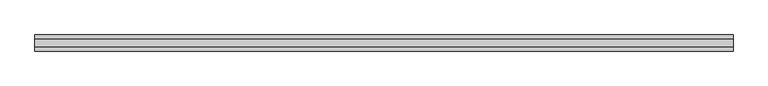
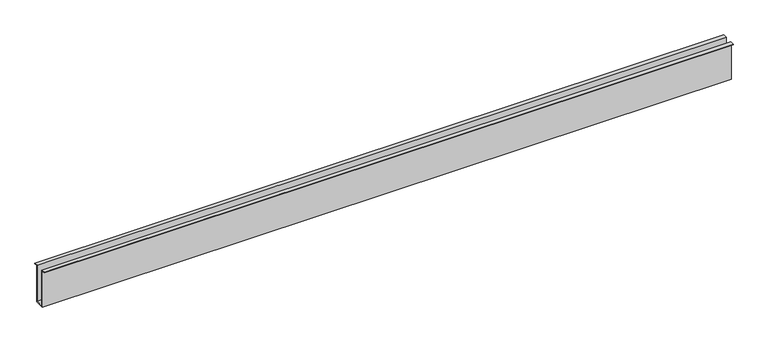
"""IFC4 building model written with IfcOpenShell, lengths in millimetres: railing geometry, ML_Perfil U de embutir1 : ML_Perfil U de embutir."""

import ifcopenshell
import ifcopenshell.guid

model = None  # the IFC model being written
_history = None  # IfcOwnerHistory: only IFC2X3 demands one
_inside = {}  # id of a spatial element -> (the spatial element, [elements in it])
_under = {}  # id of a project, library or spatial element -> (it, [spatial elements below it])
_declared = {}  # id of a project -> (the project, [libraries it declares])
_typed = {}  # id of a type object -> (the type object, [elements of that type])
_made_of = {}  # id of a material, layer set ... -> (it, [elements and type objects made of it])


def new_model(schema):
    """Start an empty IFC model of exactly this schema.

    Asked for "IFC4X3", IfcOpenShell would pick the latest addendum, in which some entities
    have other attributes; the version numbers below select the first issue.
    IFC2X3 requires an IfcOwnerHistory on every rooted entity: one is made here for all.
    """
    global model, _history
    if schema == "IFC4X3":
        model = ifcopenshell.file(schema_version=(4, 3, 0, 0))
    else:
        model = ifcopenshell.file(schema=schema)
    _inside.clear()
    _under.clear()
    _declared.clear()
    _typed.clear()
    _made_of.clear()
    _history = None
    if model.schema == "IFC2X3":
        org = make("IfcOrganization", Name="unknown")
        user = make(
            "IfcPersonAndOrganization",
            ThePerson=make("IfcPerson", FamilyName="unknown"),
            TheOrganization=org,
        )
        app = make(
            "IfcApplication",
            ApplicationDeveloper=org,
            Version="unknown",
            ApplicationFullName="unknown",
            ApplicationIdentifier="unknown",
        )
        _history = make(
            "IfcOwnerHistory",
            OwningUser=user,
            OwningApplication=app,
            ChangeAction="ADDED",
            CreationDate=0,
        )
    return model


def make(cls, **values):
    """One entity of the class cls with the attributes given. An attribute that is None is left unset."""
    return model.create_entity(
        cls, **{name: value for name, value in values.items() if value is not None}
    )


def rooted(cls, **values):
    """An entity with a GlobalId (a new one), such as an element, a storey or a relation."""
    return make(cls, GlobalId=ifcopenshell.guid.new(), OwnerHistory=_history, **values)


def si_unit(unit_type, name, prefix=None):
    """IfcSIUnit, for example si_unit("LENGTHUNIT", "METRE", prefix="MILLI")."""
    return make("IfcSIUnit", UnitType=unit_type, Prefix=prefix, Name=name)


def assignment(units):
    """IfcUnitAssignment: the units of a project."""
    return None if units is None else make("IfcUnitAssignment", Units=units)


def point(xyz):
    """IfcCartesianPoint."""
    return None if xyz is None else make("IfcCartesianPoint", Coordinates=xyz)


def direction(xyz):
    """IfcDirection."""
    return None if xyz is None else make("IfcDirection", DirectionRatios=xyz)


def frame(location, z_axis=None, x_axis=None):
    """IfcAxis2Placement3D, a coordinate frame: its origin and axes. An axis left out is left unset."""
    return make(
        "IfcAxis2Placement3D",
        Location=point(location),
        Axis=direction(z_axis),
        RefDirection=direction(x_axis),
    )


def origin():
    """The frame at (0, 0, 0) with its axes left unset."""
    return frame((0.0, 0.0, 0.0))


def place(relative_to, where):
    """IfcLocalPlacement: puts the frame where relative to a parent placement (None: the world)."""
    return make(
        "IfcLocalPlacement", PlacementRelTo=relative_to, RelativePlacement=where
    )


def context(
    kind, dimensions, precision=None, world=None, true_north=None, identifier=None
):
    """IfcGeometricRepresentationContext, for example the 3D "Model" context."""
    return make(
        "IfcGeometricRepresentationContext",
        ContextIdentifier=identifier,
        ContextType=kind,
        CoordinateSpaceDimension=dimensions,
        Precision=precision,
        WorldCoordinateSystem=world,
        TrueNorth=true_north,
    )


def project(units=None, contexts=None):
    """IfcProject with its units and contexts."""
    return rooted(
        "IfcProject",
        Name="project",
        RepresentationContexts=contexts,
        UnitsInContext=assignment(units),
    )


def spatial(cls, under=None, at=None, **own):
    """A site, building, storey or space (cls), placed at a placement, below another one or the project."""
    s = rooted(cls, ObjectPlacement=at, **own)
    if under is not None:
        _under.setdefault(under.id(), (under, []))[1].append(s)
    return s


def polyline(points):
    """IfcPolyline through the points."""
    return make("IfcPolyline", Points=[point(p) for p in points])


def outline(outer, holes=None, kind="AREA"):
    """IfcArbitraryClosedProfileDef: a profile drawn as a closed curve; with holes, ...WithVoids."""
    if holes is None:
        return make("IfcArbitraryClosedProfileDef", ProfileType=kind, OuterCurve=outer)
    return make(
        "IfcArbitraryProfileDefWithVoids",
        ProfileType=kind,
        OuterCurve=outer,
        InnerCurves=holes,
    )


def extrude(swept, where, along, depth):
    """IfcExtrudedAreaSolid: the profile swept, set in the frame where, extruded along a direction by depth."""
    return make(
        "IfcExtrudedAreaSolid",
        SweptArea=swept,
        Position=where,
        ExtrudedDirection=direction(along),
        Depth=depth,
    )


def shape(context_of_items, identifier, shape_type, items):
    """IfcShapeRepresentation: the items that make up one representation, for example the "Body"."""
    return make(
        "IfcShapeRepresentation",
        ContextOfItems=context_of_items,
        RepresentationIdentifier=identifier,
        RepresentationType=shape_type,
        Items=items,
    )


def source(mapping_origin, context_of_items, identifier, shape_type, items):
    """IfcRepresentationMap: a shape defined once, which mapped items show again and again."""
    return make(
        "IfcRepresentationMap",
        MappingOrigin=mapping_origin,
        MappedRepresentation=shape(context_of_items, identifier, shape_type, items),
    )


def transform(
    local_origin,
    x_axis=None,
    y_axis=None,
    z_axis=None,
    scale=None,
    scale2=None,
    scale3=None,
    uniform=True,
):
    """IfcCartesianTransformationOperator3D, or its non-uniform kind. x_axis, y_axis, z_axis: its Axis1, 2, 3."""
    if uniform:
        return make(
            "IfcCartesianTransformationOperator3D",
            Axis1=direction(x_axis),
            Axis2=direction(y_axis),
            LocalOrigin=point(local_origin),
            Scale=scale,
            Axis3=direction(z_axis),
        )
    return make(
        "IfcCartesianTransformationOperator3DnonUniform",
        Axis1=direction(x_axis),
        Axis2=direction(y_axis),
        LocalOrigin=point(local_origin),
        Scale=scale,
        Axis3=direction(z_axis),
        Scale2=scale2,
        Scale3=scale3,
    )


def mapped(mapping_source, mapping_target):
    """IfcMappedItem: shows the shape of a source again, moved by a transform."""
    return make(
        "IfcMappedItem", MappingSource=mapping_source, MappingTarget=mapping_target
    )


def made_of(thing, what):
    """Note that an element or type object is made of a material, layer set ...; save() writes the relation."""
    if what is not None:
        _made_of.setdefault(what.id(), (what, []))[1].append(thing)
    return thing


def element(
    cls,
    number,
    at=None,
    inside=None,
    cuts=None,
    type_object=None,
    material=None,
    context=None,
    identifier="Body",
    shape_type=None,
    held_by="IfcProductDefinitionShape",
    body=None,
    shapes=None,
    **own,
):
    """One element of the class cls, such as IfcWall. Its Tag is "e" and its number.

    at: its placement. inside: the storey or other place that contains it. cuts: it is an
    opening in that element (IfcRelVoidsElement). A single representation is given by context,
    identifier, shape_type and body (its items); several are given by shapes. held_by: the class
    of the entity that holds the representations. save() writes the other relations.
    """
    e = rooted(cls, Tag="e%d" % number, ObjectPlacement=at, **own)
    if body is not None:
        shapes = [shape(context, identifier, shape_type, body)]
    if shapes is not None:
        e.Representation = make(held_by, Representations=shapes)
    if inside is not None:
        _inside.setdefault(inside.id(), (inside, []))[1].append(e)
    if cuts is not None:
        rooted(
            "IfcRelVoidsElement", RelatingBuildingElement=cuts, RelatedOpeningElement=e
        )
    if type_object is not None:
        _typed.setdefault(type_object.id(), (type_object, []))[1].append(e)
    return made_of(e, material)


def aggregate(whole, parts):
    """IfcRelAggregates: a whole, such as a stair, and the parts it consists of."""
    return rooted("IfcRelAggregates", RelatingObject=whole, RelatedObjects=parts)


def save(model, path):
    """Write the relations noted so far, then the file.

    IfcRelAggregates (storeys below a building ...), IfcRelContainedInSpatialStructure (elements
    in a storey), IfcRelDefinesByType, IfcRelAssociatesMaterial and IfcRelDeclares: one each for
    every whole, place, type object, material and project.
    """
    for whole, parts in _under.values():
        aggregate(whole, parts)
    for where, things in _inside.values():
        rooted(
            "IfcRelContainedInSpatialStructure",
            RelatedElements=things,
            RelatingStructure=where,
        )
    for kind, things in _typed.values():
        rooted("IfcRelDefinesByType", RelatedObjects=things, RelatingType=kind)
    for what, things in _made_of.values():
        rooted("IfcRelAssociatesMaterial", RelatedObjects=things, RelatingMaterial=what)
    for by, libraries in _declared.values():
        rooted("IfcRelDeclares", RelatingContext=by, RelatedDefinitions=libraries)
    model.write(path)


def railing_4d275163(model_context):
    return source(origin(), model_context, "Body", "SweptSolid", [
        extrude(outline(polyline([(1832.4523952, 3702.0), (1832.4523952, 3594.0), (1856.4523952, 3594.0), (1856.4523952, 3702.0), (1866.9523952, 3702.0), (1866.9523952, 3700.0), (1858.4523952, 3700.0), (1858.4523952, 3592.0), (1830.4523952, 3592.0), (1830.4523952, 3700.0), (1821.9523952, 3700.0), (1821.9523952, 3702.0), (1832.4523952, 3702.0)])), frame((-12226.1487231, 0.0, 0.0), z_axis=(1.0, 0.0, 0.0), x_axis=(0.0, 1.0, 0.0)), (0.0, 0.0, 1.0), 1950.0),
    ])


if __name__ == "__main__":
    model = new_model("IFC4")
    model_context = context("Model", 3, world=origin())
    ifc_project = project(units=[si_unit("LENGTHUNIT", "METRE", prefix="MILLI")], contexts=[model_context])
    site = spatial("IfcSite", under=ifc_project)
    building = spatial("IfcBuilding", under=site)
    placement = place(None, origin())
    railing_shape = railing_4d275163(model_context)
    element("IfcRailing", 1, ObjectType="ML_Perfil U de embutir1 : ML_Perfil U de embutir", at=placement, inside=building, context=model_context, shape_type="MappedRepresentation", body=[
        mapped(railing_shape, transform((0.0, 0.0, 0.0), x_axis=(1.0, 0.0, 0.0), y_axis=(0.0, 1.0, 0.0), z_axis=(0.0, 0.0, 1.0))),
    ])
    save(model, "model.ifc")

# Revit data of these elements
# Type "ML_Perfil U de embutir1 : ML_Perfil U de embutir"
#   ME_Compr [instance default] = 1.95 m
#   ME_Material Perfil [instance default] = .ALUMÍNIO COM PINTURA ELETROSTÁTICA BRANCA
# Element 1 (IfcRailing, "ML_Perfil U de embutir1 : ML_Perfil U de embutir")
#   Materials on its faces: ".ALUMÍNIO COM PINTURA ELETROSTÁTICA BRANCA"
# Materials
#   ".ALUMÍNIO COM PINTURA ELETROSTÁTICA BRANCA": class "CC_METAIS", colour RGB 241 241 241, transparency 0, Cost = 0
